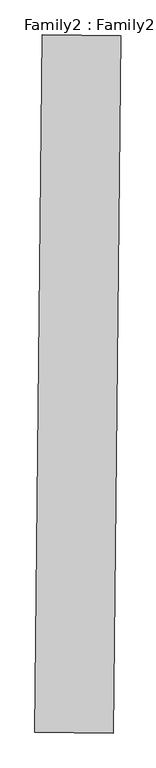
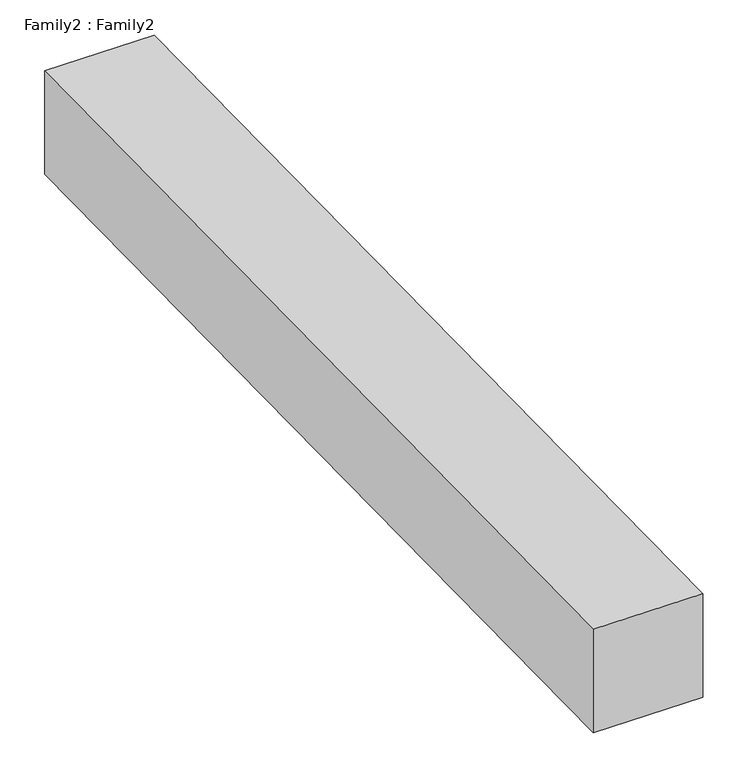
"""IFC4 building model written with IfcOpenShell, lengths in millimetres: proxy geometry, Family2 : Family2."""

from ifc_helpers import new_model, si_unit, origin, place, context, project, spatial, faceted_brep, source, transform, mapped, element, save


def family2_family2_5112019e(model_context):
    return source(origin(), model_context, "Body", "Brep", [
        faceted_brep([(-3952.5660924, -6961.2601034, 1.0945136), (-3952.5660924, -6961.2601034, 201.0945136), (-3934.2767021, -5186.3400192, 202.060409), (-3934.2767021, -5186.3400192, 2.060409), (-3752.5749025, -6963.1373161, 201.0945136), (-3734.2855121, -5188.2172318, 202.060409), (-3752.5749025, -6963.1373161, 1.0945136), (-3734.2855121, -5188.2172318, 2.060409)], [[[0, 1, 2, 3]], [[1, 4, 5, 2]], [[4, 6, 7, 5]], [[6, 0, 3, 7]], [[3, 2, 5, 7]], [[0, 6, 4, 1]]]),
    ])


if __name__ == "__main__":
    model = new_model("IFC4")
    model_context = context("Model", 3, world=origin())
    ifc_project = project(units=[si_unit("LENGTHUNIT", "METRE", prefix="MILLI")], contexts=[model_context])
    site = spatial("IfcSite", under=ifc_project)
    building = spatial("IfcBuilding", under=site)
    placement = place(None, origin())
    family2_family2_shape = family2_family2_5112019e(model_context)
    element("IfcBuildingElementProxy", 1, Name="Family2 : Family2", ObjectType="Family2 : Family2", at=placement, inside=building, context=model_context, shape_type="MappedRepresentation", body=[
        mapped(family2_family2_shape, transform((0.0, 0.0, 0.0), x_axis=(1.0, 0.0, 0.0), y_axis=(0.0, 1.0, 0.0), z_axis=(0.0, 0.0, 1.0))),
    ])
    save(model, "model.ifc")

# Revit data of these elements
# Type "Family2 : Family2"
#   Default Elevation = 0
